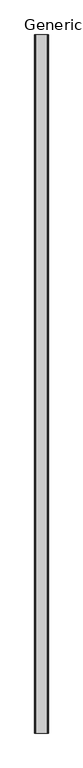
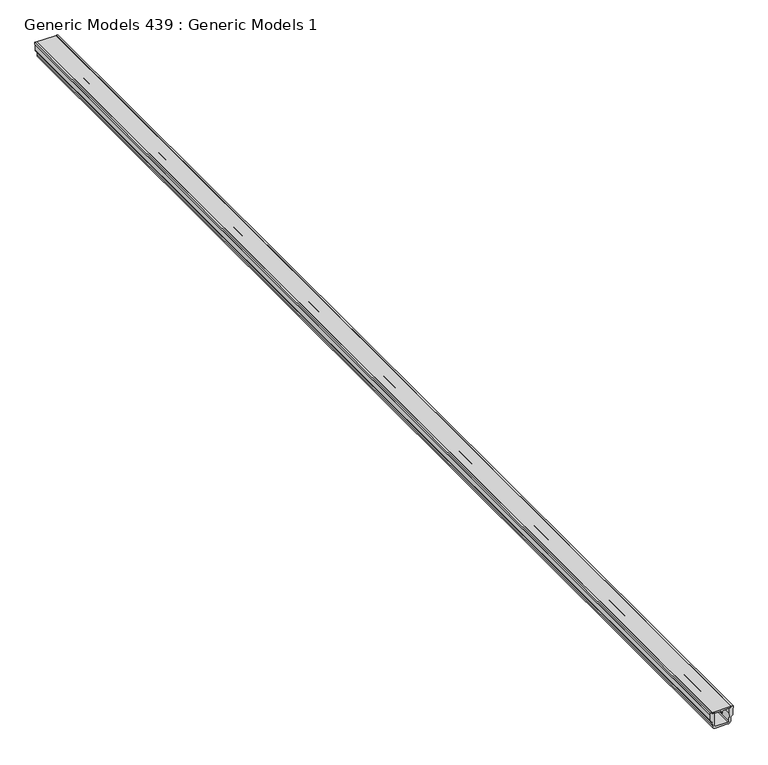
"""IFC4 building model written with IfcOpenShell, lengths in millimetres: proxy geometry, Generic Models 439 : Generic Models 1."""

from ifc_helpers import new_model, si_unit, point, frame, frame_2d, origin, place, context, project, spatial, polyline, circle_curve, trimmed, segment, composite_curve, outline, extrude, source, transform, mapped, element, save


def generic_models_439_generic_models_1_a3366f08(model_context):
    return source(origin(), model_context, "Body", "SweptSolid", [
        extrude(outline(composite_curve([segment(polyline([(126745.571071, -6636.7184448), (126745.571071, -6551.7144873)]), True, "CONTINUOUS"), segment(trimmed(circle_curve(frame_2d((126764.8232791, -6551.7144873)), 19.2522081), [point((126745.571071, -6551.7144873))], [point((126764.8232791, -6532.4622792))], False, "CARTESIAN"), True, "CONTINUOUS"), segment(polyline([(126764.8232791, -6532.4622792), (126791.1626529, -6531.3292916)]), True, "CONTINUOUS"), segment(trimmed(circle_curve(frame_2d((126790.8868635, -6524.9178177)), 6.4174027), [point((126791.1626529, -6531.3292916))], [point((126797.1466767, -6526.3312516))], True, "CARTESIAN"), True, "CONTINUOUS"), segment(trimmed(circle_curve(frame_2d((126806.5363966, -6528.4514025)), 9.626104), [point((126797.1466767, -6526.3312516))], [point((126806.5363966, -6518.8252984))], False, "CARTESIAN"), True, "CONTINUOUS"), segment(polyline([(126806.5363966, -6518.8252984), (126846.6451635, -6518.8252984)]), True, "CONTINUOUS"), segment(trimmed(circle_curve(frame_2d((126846.6451635, -6517.2209478)), 1.6043507), [point((126846.6451635, -6518.8252984))], [point((126848.2495142, -6517.2209478))], True, "CARTESIAN"), True, "CONTINUOUS"), segment(polyline([(126848.2495142, -6517.2209478), (126862.6886702, -6517.2209478), (126862.6886702, -6528.1150807), (126856.2712675, -6528.4514025), (126856.2712675, -6543.0887292), (126816.1625007, -6543.0887292), (126764.2722099, -6545.3207888)]), True, "CONTINUOUS"), segment(trimmed(circle_curve(frame_2d((126764.8232791, -6551.7144873)), 6.4174027), [point((126764.2722099, -6545.3207888))], [point((126758.4058764, -6551.7144873))], True, "CARTESIAN"), True, "CONTINUOUS"), segment(polyline([(126758.4058764, -6551.7144873), (126758.4058764, -6636.7184448)]), True, "CONTINUOUS"), segment(trimmed(circle_curve(frame_2d((126764.8232791, -6636.7184448)), 6.4174027), [point((126758.4058764, -6636.7184448))], [point((126764.2722099, -6643.1121433))], True, "CARTESIAN"), True, "CONTINUOUS"), segment(polyline([(126764.2722099, -6643.1121433), (126816.1625007, -6645.3442029), (126856.2712675, -6645.3442029), (126856.2712675, -6659.9815296), (126862.6886702, -6660.3178514), (126862.6886702, -6671.2119843), (126848.2495142, -6671.2119843)]), True, "CONTINUOUS"), segment(trimmed(circle_curve(frame_2d((126846.6451635, -6671.2119843)), 1.6043507), [point((126848.2495142, -6671.2119843))], [point((126846.6451635, -6669.6076337))], True, "CARTESIAN"), True, "CONTINUOUS"), segment(polyline([(126846.6451635, -6669.6076337), (126806.5363966, -6669.6076337)]), True, "CONTINUOUS"), segment(trimmed(circle_curve(frame_2d((126806.5363966, -6659.9815296)), 9.626104), [point((126806.5363966, -6669.6076337))], [point((126797.1466767, -6662.1016805))], False, "CARTESIAN"), True, "CONTINUOUS"), segment(trimmed(circle_curve(frame_2d((126790.8868635, -6663.5151144)), 6.4174027), [point((126797.1466767, -6662.1016805))], [point((126791.1626529, -6657.1036405))], True, "CARTESIAN"), True, "CONTINUOUS"), segment(polyline([(126791.1626529, -6657.1036405), (126764.8232791, -6655.9706529)]), True, "CONTINUOUS"), segment(trimmed(circle_curve(frame_2d((126764.8232791, -6636.7184448)), 19.2522081), [point((126764.8232791, -6655.9706529))], [point((126745.571071, -6636.7184448))], False, "CARTESIAN"), True, "CONTINUOUS")], self_intersect=False)), frame((0.0, -5493.3230338, 0.0), z_axis=(0.0, 1.0, 0.0), x_axis=(0.0, 0.0, 1.0)), (0.0, 0.0, 1.0), 7886.7),
        extrude(outline(composite_curve([segment(polyline([(126848.6261398, -6598.0461702), (126837.0190595, -6597.234524), (126837.0190595, -6591.1984081), (126848.6261398, -6590.3867619)]), True, "CONTINUOUS"), segment(trimmed(circle_curve(frame_2d((126848.4041696, -6587.2124402)), 3.1820731), [point((126848.6261398, -6590.3867619))], [point((126851.5641479, -6587.5867749))], True, "CARTESIAN"), True, "CONTINUOUS"), segment(polyline([(126851.5641479, -6587.5867749), (126857.0650175, -6541.1507219), (126857.0650175, -6530.3504763), (126862.6886702, -6530.0557532), (126862.6886702, -6658.3771789), (126857.0650175, -6658.0824558), (126857.0650175, -6647.2822102), (126851.5641479, -6600.8461572)]), True, "CONTINUOUS"), segment(trimmed(circle_curve(frame_2d((126848.4041696, -6601.2204919)), 3.1820731), [point((126851.5641479, -6600.8461572))], [point((126848.6261398, -6598.0461702))], True, "CARTESIAN"), True, "CONTINUOUS")], self_intersect=False)), frame((0.0, -5493.3230338, 0.0), z_axis=(0.0, 1.0, 0.0), x_axis=(0.0, 0.0, 1.0)), (0.0, 0.0, 1.0), 7886.7),
    ])


if __name__ == "__main__":
    model = new_model("IFC4")
    model_context = context("Model", 3, world=origin())
    ifc_project = project(units=[si_unit("LENGTHUNIT", "METRE", prefix="MILLI")], contexts=[model_context])
    site = spatial("IfcSite", under=ifc_project)
    building = spatial("IfcBuilding", under=site)
    placement = place(None, origin())
    generic_models_439_generic_models_1_shape = generic_models_439_generic_models_1_a3366f08(model_context)
    element("IfcBuildingElementProxy", 1, Name="Generic Models 439 : Generic Models 1", ObjectType="Generic Models 439 : Generic Models 1", at=placement, inside=building, context=model_context, shape_type="MappedRepresentation", body=[
        mapped(generic_models_439_generic_models_1_shape, transform((0.0, 0.0, 0.0), x_axis=(1.0, 0.0, 0.0), y_axis=(0.0, 1.0, 0.0), z_axis=(0.0, 0.0, 1.0))),
    ])
    save(model, "model.ifc")

# Revit data of these elements
# Element 1 (IfcBuildingElementProxy, "Generic Models 439 : Generic Models 1")
#   Materials on its faces: "_TRENCH DRAIN WITH MEMBRANE CLAMPS"
# Materials
#   "_TRENCH DRAIN WITH MEMBRANE CLAMPS": class "Generic", colour RGB 253 192 103, transparency 0, Cost = 0
